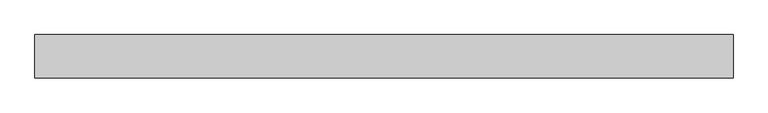
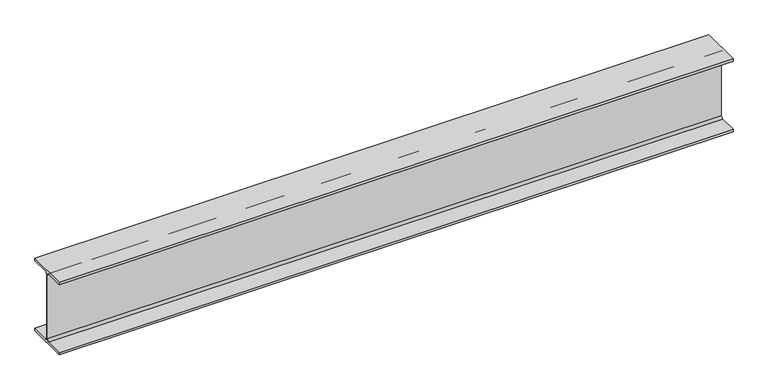
"""IFC4 building model written with IfcOpenShell, lengths in millimetres: beam geometry, Steel Beam_H-KSD3502 : H_SB_ASB_H-194x150x6x9."""

import ifcopenshell
import ifcopenshell.guid

model = None  # the IFC model being written
_history = None  # IfcOwnerHistory: only IFC2X3 demands one
_inside = {}  # id of a spatial element -> (the spatial element, [elements in it])
_under = {}  # id of a project, library or spatial element -> (it, [spatial elements below it])
_declared = {}  # id of a project -> (the project, [libraries it declares])
_typed = {}  # id of a type object -> (the type object, [elements of that type])
_made_of = {}  # id of a material, layer set ... -> (it, [elements and type objects made of it])


def new_model(schema):
    """Start an empty IFC model of exactly this schema.

    Asked for "IFC4X3", IfcOpenShell would pick the latest addendum, in which some entities
    have other attributes; the version numbers below select the first issue.
    IFC2X3 requires an IfcOwnerHistory on every rooted entity: one is made here for all.
    """
    global model, _history
    if schema == "IFC4X3":
        model = ifcopenshell.file(schema_version=(4, 3, 0, 0))
    else:
        model = ifcopenshell.file(schema=schema)
    _inside.clear()
    _under.clear()
    _declared.clear()
    _typed.clear()
    _made_of.clear()
    _history = None
    if model.schema == "IFC2X3":
        org = make("IfcOrganization", Name="unknown")
        user = make(
            "IfcPersonAndOrganization",
            ThePerson=make("IfcPerson", FamilyName="unknown"),
            TheOrganization=org,
        )
        app = make(
            "IfcApplication",
            ApplicationDeveloper=org,
            Version="unknown",
            ApplicationFullName="unknown",
            ApplicationIdentifier="unknown",
        )
        _history = make(
            "IfcOwnerHistory",
            OwningUser=user,
            OwningApplication=app,
            ChangeAction="ADDED",
            CreationDate=0,
        )
    return model


def make(cls, **values):
    """One entity of the class cls with the attributes given. An attribute that is None is left unset."""
    return model.create_entity(
        cls, **{name: value for name, value in values.items() if value is not None}
    )


def rooted(cls, **values):
    """An entity with a GlobalId (a new one), such as an element, a storey or a relation."""
    return make(cls, GlobalId=ifcopenshell.guid.new(), OwnerHistory=_history, **values)


def si_unit(unit_type, name, prefix=None):
    """IfcSIUnit, for example si_unit("LENGTHUNIT", "METRE", prefix="MILLI")."""
    return make("IfcSIUnit", UnitType=unit_type, Prefix=prefix, Name=name)


def assignment(units):
    """IfcUnitAssignment: the units of a project."""
    return None if units is None else make("IfcUnitAssignment", Units=units)


def point(xyz):
    """IfcCartesianPoint."""
    return None if xyz is None else make("IfcCartesianPoint", Coordinates=xyz)


def direction(xyz):
    """IfcDirection."""
    return None if xyz is None else make("IfcDirection", DirectionRatios=xyz)


def frame(location, z_axis=None, x_axis=None):
    """IfcAxis2Placement3D, a coordinate frame: its origin and axes. An axis left out is left unset."""
    return make(
        "IfcAxis2Placement3D",
        Location=point(location),
        Axis=direction(z_axis),
        RefDirection=direction(x_axis),
    )


def frame_2d(location, x_axis=None):
    """IfcAxis2Placement2D, a coordinate frame in the plane: its origin and x axis."""
    return make(
        "IfcAxis2Placement2D", Location=point(location), RefDirection=direction(x_axis)
    )


def origin():
    """The frame at (0, 0, 0) with its axes left unset."""
    return frame((0.0, 0.0, 0.0))


def place(relative_to, where):
    """IfcLocalPlacement: puts the frame where relative to a parent placement (None: the world)."""
    return make(
        "IfcLocalPlacement", PlacementRelTo=relative_to, RelativePlacement=where
    )


def context(
    kind, dimensions, precision=None, world=None, true_north=None, identifier=None
):
    """IfcGeometricRepresentationContext, for example the 3D "Model" context."""
    return make(
        "IfcGeometricRepresentationContext",
        ContextIdentifier=identifier,
        ContextType=kind,
        CoordinateSpaceDimension=dimensions,
        Precision=precision,
        WorldCoordinateSystem=world,
        TrueNorth=true_north,
    )


def project(units=None, contexts=None):
    """IfcProject with its units and contexts."""
    return rooted(
        "IfcProject",
        Name="project",
        RepresentationContexts=contexts,
        UnitsInContext=assignment(units),
    )


def spatial(cls, under=None, at=None, **own):
    """A site, building, storey or space (cls), placed at a placement, below another one or the project."""
    s = rooted(cls, ObjectPlacement=at, **own)
    if under is not None:
        _under.setdefault(under.id(), (under, []))[1].append(s)
    return s


def polyline(points):
    """IfcPolyline through the points."""
    return make("IfcPolyline", Points=[point(p) for p in points])


def circle_curve(where, radius):
    """IfcCircle in the frame where."""
    return make("IfcCircle", Position=where, Radius=radius)


def trimmed(basis, trim1, trim2, sense, master):
    """IfcTrimmedCurve: the piece of a basis curve between two trims."""
    return make(
        "IfcTrimmedCurve",
        BasisCurve=basis,
        Trim1=trim1,
        Trim2=trim2,
        SenseAgreement=sense,
        MasterRepresentation=master,
    )


def segment(curve, same_sense, transition):
    """IfcCompositeCurveSegment."""
    return make(
        "IfcCompositeCurveSegment",
        Transition=transition,
        SameSense=same_sense,
        ParentCurve=curve,
    )


def composite_curve(segments, self_intersect=None):
    """IfcCompositeCurve: segments joined end to end."""
    return make("IfcCompositeCurve", Segments=segments, SelfIntersect=self_intersect)


def outline(outer, holes=None, kind="AREA"):
    """IfcArbitraryClosedProfileDef: a profile drawn as a closed curve; with holes, ...WithVoids."""
    if holes is None:
        return make("IfcArbitraryClosedProfileDef", ProfileType=kind, OuterCurve=outer)
    return make(
        "IfcArbitraryProfileDefWithVoids",
        ProfileType=kind,
        OuterCurve=outer,
        InnerCurves=holes,
    )


def extrude(swept, where, along, depth):
    """IfcExtrudedAreaSolid: the profile swept, set in the frame where, extruded along a direction by depth."""
    return make(
        "IfcExtrudedAreaSolid",
        SweptArea=swept,
        Position=where,
        ExtrudedDirection=direction(along),
        Depth=depth,
    )


def shape(context_of_items, identifier, shape_type, items):
    """IfcShapeRepresentation: the items that make up one representation, for example the "Body"."""
    return make(
        "IfcShapeRepresentation",
        ContextOfItems=context_of_items,
        RepresentationIdentifier=identifier,
        RepresentationType=shape_type,
        Items=items,
    )


def source(mapping_origin, context_of_items, identifier, shape_type, items):
    """IfcRepresentationMap: a shape defined once, which mapped items show again and again."""
    return make(
        "IfcRepresentationMap",
        MappingOrigin=mapping_origin,
        MappedRepresentation=shape(context_of_items, identifier, shape_type, items),
    )


def transform(
    local_origin,
    x_axis=None,
    y_axis=None,
    z_axis=None,
    scale=None,
    scale2=None,
    scale3=None,
    uniform=True,
):
    """IfcCartesianTransformationOperator3D, or its non-uniform kind. x_axis, y_axis, z_axis: its Axis1, 2, 3."""
    if uniform:
        return make(
            "IfcCartesianTransformationOperator3D",
            Axis1=direction(x_axis),
            Axis2=direction(y_axis),
            LocalOrigin=point(local_origin),
            Scale=scale,
            Axis3=direction(z_axis),
        )
    return make(
        "IfcCartesianTransformationOperator3DnonUniform",
        Axis1=direction(x_axis),
        Axis2=direction(y_axis),
        LocalOrigin=point(local_origin),
        Scale=scale,
        Axis3=direction(z_axis),
        Scale2=scale2,
        Scale3=scale3,
    )


def mapped(mapping_source, mapping_target):
    """IfcMappedItem: shows the shape of a source again, moved by a transform."""
    return make(
        "IfcMappedItem", MappingSource=mapping_source, MappingTarget=mapping_target
    )


def made_of(thing, what):
    """Note that an element or type object is made of a material, layer set ...; save() writes the relation."""
    if what is not None:
        _made_of.setdefault(what.id(), (what, []))[1].append(thing)
    return thing


def element(
    cls,
    number,
    at=None,
    inside=None,
    cuts=None,
    type_object=None,
    material=None,
    context=None,
    identifier="Body",
    shape_type=None,
    held_by="IfcProductDefinitionShape",
    body=None,
    shapes=None,
    **own,
):
    """One element of the class cls, such as IfcWall. Its Tag is "e" and its number.

    at: its placement. inside: the storey or other place that contains it. cuts: it is an
    opening in that element (IfcRelVoidsElement). A single representation is given by context,
    identifier, shape_type and body (its items); several are given by shapes. held_by: the class
    of the entity that holds the representations. save() writes the other relations.
    """
    e = rooted(cls, Tag="e%d" % number, ObjectPlacement=at, **own)
    if body is not None:
        shapes = [shape(context, identifier, shape_type, body)]
    if shapes is not None:
        e.Representation = make(held_by, Representations=shapes)
    if inside is not None:
        _inside.setdefault(inside.id(), (inside, []))[1].append(e)
    if cuts is not None:
        rooted(
            "IfcRelVoidsElement", RelatingBuildingElement=cuts, RelatedOpeningElement=e
        )
    if type_object is not None:
        _typed.setdefault(type_object.id(), (type_object, []))[1].append(e)
    return made_of(e, material)


def aggregate(whole, parts):
    """IfcRelAggregates: a whole, such as a stair, and the parts it consists of."""
    return rooted("IfcRelAggregates", RelatingObject=whole, RelatedObjects=parts)


def save(model, path):
    """Write the relations noted so far, then the file.

    IfcRelAggregates (storeys below a building ...), IfcRelContainedInSpatialStructure (elements
    in a storey), IfcRelDefinesByType, IfcRelAssociatesMaterial and IfcRelDeclares: one each for
    every whole, place, type object, material and project.
    """
    for whole, parts in _under.values():
        aggregate(whole, parts)
    for where, things in _inside.values():
        rooted(
            "IfcRelContainedInSpatialStructure",
            RelatedElements=things,
            RelatingStructure=where,
        )
    for kind, things in _typed.values():
        rooted("IfcRelDefinesByType", RelatedObjects=things, RelatingType=kind)
    for what, things in _made_of.values():
        rooted("IfcRelAssociatesMaterial", RelatedObjects=things, RelatingMaterial=what)
    for by, libraries in _declared.values():
        rooted("IfcRelDeclares", RelatingContext=by, RelatedDefinitions=libraries)
    model.write(path)


def beam_c6f56534(model_context):
    return source(origin(), model_context, "Body", "SweptSolid", [
        extrude(outline(composite_curve([segment(polyline([(-82.5, -141.5), (-11.9, -141.5)]), True, "CONTINUOUS"), segment(trimmed(circle_curve(frame_2d((-11.9, -132.6)), 8.9), [point((-11.9, -141.5))], [point((-3.0, -132.6))], True, "CARTESIAN"), True, "CONTINUOUS"), segment(polyline([(-3.0, -132.6), (-3.0, 132.6)]), True, "CONTINUOUS"), segment(trimmed(circle_curve(frame_2d((-11.9, 132.6)), 8.9), [point((-3.0, 132.6))], [point((-11.9, 141.5))], True, "CARTESIAN"), True, "CONTINUOUS"), segment(polyline([(-11.9, 141.5), (-82.5, 141.5), (-82.5, 151.7), (82.5, 151.7), (82.5, 141.5), (11.9, 141.5)]), True, "CONTINUOUS"), segment(trimmed(circle_curve(frame_2d((11.9, 132.6)), 8.9), [point((11.9, 141.5))], [point((3.0, 132.6))], True, "CARTESIAN"), True, "CONTINUOUS"), segment(polyline([(3.0, 132.6), (3.0, -132.6)]), True, "CONTINUOUS"), segment(trimmed(circle_curve(frame_2d((11.9, -132.6)), 8.9), [point((3.0, -132.6))], [point((11.9, -141.5))], True, "CARTESIAN"), True, "CONTINUOUS"), segment(polyline([(11.9, -141.5), (82.5, -141.5), (82.5, -151.7), (-82.5, -151.7), (-82.5, -141.5)]), True, "CONTINUOUS")], self_intersect=False)), frame((-1106.6961534, 0.0, 0.0), z_axis=(1.0, 0.0, 0.0), x_axis=(0.0, 1.0, 0.0)), (0.0, 0.0, 1.0), 2655.7235444),
    ])


if __name__ == "__main__":
    model = new_model("IFC4")
    model_context = context("Model", 3, world=origin())
    ifc_project = project(units=[si_unit("LENGTHUNIT", "METRE", prefix="MILLI")], contexts=[model_context])
    site = spatial("IfcSite", under=ifc_project)
    building = spatial("IfcBuilding", under=site)
    placement = place(None, origin())
    beam_shape = beam_c6f56534(model_context)
    element("IfcBeam", 1, ObjectType="Steel Beam_H-KSD3502 : H_SB_ASB_H-194x150x6x9", at=placement, inside=building, context=model_context, shape_type="MappedRepresentation", body=[
        mapped(beam_shape, transform((0.0, 0.0, 0.0), x_axis=(1.0, 0.0, 0.0), y_axis=(0.0, 1.0, 0.0), z_axis=(0.0, 0.0, 1.0))),
    ])
    save(model, "model.ifc")

# Revit data of these elements
# Type "Steel Beam_H-KSD3502 : H_SB_ASB_H-194x150x6x9"
#   Width = 15.0 cm
#   Web Thickness = 0.6 cm
#   Web Fillet = 1.3 cm
#   Warping Constant = 43316.0 cm⁶
#   Torsional Moment of Inertia = 8.622 cm⁴
#   Torsional Modulus = 1.0 cm³
#   Section Area = 39.01 cm²
#   Plastic Modulus weak axis = 104.0 cm³
#   Plastic Modulus strong axis = 309.0 cm³
#   Perimeter = 0.95 m²/m
#   Nominal Weight = 30.60 kgf/m
#   Moment of Inertia weak axis = 507.00 cm⁴
#   Moment of Inertia strong axis = 2690.00 cm⁴
#   Height = 19.4 cm
#   Flange Thickness = 0.9 cm
#   Elastic Modulus weak axis = 67.6 cm³
#   Elastic Modulus strong axis = 277.0 cm³
#   Centroid Vertical = 9.7 cm
#   Centroid Horizontal = 7.5 cm
#   Length [instance default] = 1.5240 m
#   Structural Material [instance default] = Steel, 45-345
#   Assembly Code = ""
# Element 1 (IfcBeam, "Steel Beam_H-KSD3502 : H_SB_ASB_H-194x150x6x9")
#   Structural Material = none
# Materials
#   "Steel, 45-345": class "Metal", colour RGB 189 187 185, transparency 0, Description = "Steel 345 MPa", Cost = 0
